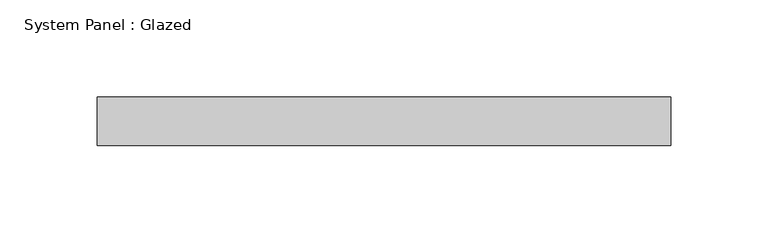
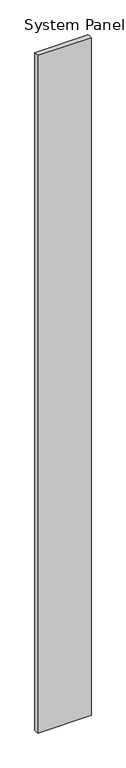
"""IFC4 building model written with IfcOpenShell, lengths in millimetres: plate geometry, System Panel : Glazed."""

from ifc_helpers import new_model, si_unit, origin, origin_with_axes, place, context, project, spatial, polyline, outline, extrude, source, transform, mapped, element, save


def system_panel_glazed_30460a32(model_context):
    return source(origin(), model_context, "Body", "SweptSolid", [
        extrude(outline(polyline([(147.4999998, 24.5), (-147.4999998, 24.5), (-147.4999998, 49.5), (147.4999998, 49.5), (147.4999998, 24.5)])), origin_with_axes(), (0.0, 0.0, 1.0), 3950.0),
    ])


if __name__ == "__main__":
    model = new_model("IFC4")
    model_context = context("Model", 3, world=origin())
    ifc_project = project(units=[si_unit("LENGTHUNIT", "METRE", prefix="MILLI")], contexts=[model_context])
    site = spatial("IfcSite", under=ifc_project)
    building = spatial("IfcBuilding", under=site)
    placement = place(None, origin())
    system_panel_glazed_shape = system_panel_glazed_30460a32(model_context)
    element("IfcPlate", 1, ObjectType="System Panel : Glazed", at=placement, inside=building, context=model_context, shape_type="MappedRepresentation", body=[
        mapped(system_panel_glazed_shape, transform((0.0, 0.0, 0.0), x_axis=(1.0, 0.0, 0.0), y_axis=(0.0, 1.0, 0.0), z_axis=(0.0, 0.0, 1.0))),
    ])
    save(model, "model.ifc")

# Revit data of these elements
# Type "System Panel : Glazed"
#   Keynote = "H11"
#   Construction Type Id = "GSP4R"
#   Analytic Construction = "1/8 in Pilkington single glazing"
#   Visual Light Transmittance = 0.9
#   Solar Heat Gain Coefficient = 0.86
#   Heat Transfer Coefficient (U) = 6.7069 W/(m²·K)
#   Define Thermal Properties by = 1
# Element 1 (IfcPlate, "System Panel : Glazed")
#   Materials on its faces: "Glass"
# Materials
#   "Glass": class "Glass", colour RGB 0 128 192, transparency 0.9, Description = "Soda Lime Glass", Cost = 0
